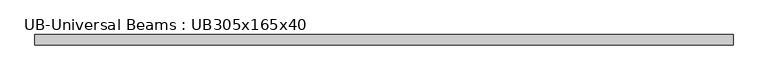
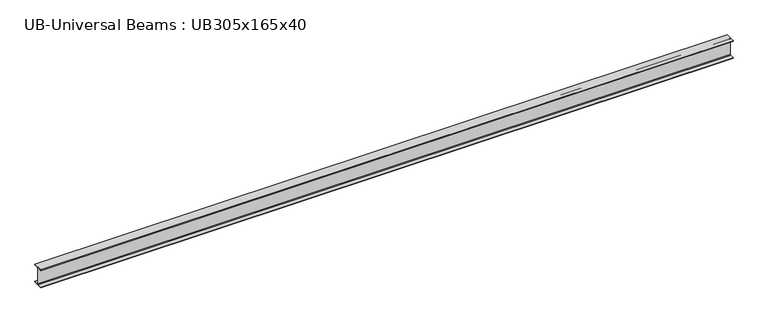
"""IFC4 building model written with IfcOpenShell, lengths in millimetres: member geometry, UB-Universal Beams : UB305x165x40."""

from ifc_helpers import new_model, si_unit, point, frame, frame_2d, origin, place, context, project, spatial, polyline, circle_curve, trimmed, segment, composite_curve, outline, extrude, source, transform, mapped, element, save


def ub_universal_beams_ub305x165x40_49d98a2e(model_context):
    return source(origin(), model_context, "Body", "SweptSolid", [
        extrude(outline(composite_curve([segment(polyline([(82.5, -141.5), (82.5, -151.7), (-82.5, -151.7), (-82.5, -141.5), (-11.9, -141.5)]), True, "CONTINUOUS"), segment(trimmed(circle_curve(frame_2d((-11.9, -132.6)), 8.9), [point((-11.9, -141.5))], [point((-3.0, -132.6))], True, "CARTESIAN"), True, "CONTINUOUS"), segment(polyline([(-3.0, -132.6), (-3.0, 132.6)]), True, "CONTINUOUS"), segment(trimmed(circle_curve(frame_2d((-11.9, 132.6)), 8.9), [point((-3.0, 132.6))], [point((-11.9, 141.5))], True, "CARTESIAN"), True, "CONTINUOUS"), segment(polyline([(-11.9, 141.5), (-82.5, 141.5), (-82.5, 151.7), (82.5, 151.7), (82.5, 141.5), (11.9, 141.5)]), True, "CONTINUOUS"), segment(trimmed(circle_curve(frame_2d((11.9, 132.6)), 8.9), [point((11.9, 141.5))], [point((3.0, 132.6))], True, "CARTESIAN"), True, "CONTINUOUS"), segment(polyline([(3.0, 132.6), (3.0, -132.6)]), True, "CONTINUOUS"), segment(trimmed(circle_curve(frame_2d((11.9, -132.6)), 8.9), [point((3.0, -132.6))], [point((11.9, -141.5))], True, "CARTESIAN"), True, "CONTINUOUS"), segment(polyline([(11.9, -141.5), (82.5, -141.5)]), True, "CONTINUOUS")], self_intersect=False)), frame((-5634.8, 0.0, 0.0), z_axis=(1.0, 0.0, 0.0), x_axis=(0.0, 1.0, 0.0)), (0.0, 0.0, 1.0), 11256.5),
    ])


if __name__ == "__main__":
    model = new_model("IFC4")
    model_context = context("Model", 3, world=origin())
    ifc_project = project(units=[si_unit("LENGTHUNIT", "METRE", prefix="MILLI")], contexts=[model_context])
    site = spatial("IfcSite", under=ifc_project)
    building = spatial("IfcBuilding", under=site)
    placement = place(None, origin())
    ub_universal_beams_ub305x165x40_shape = ub_universal_beams_ub305x165x40_49d98a2e(model_context)
    element("IfcMember", 1, ObjectType="UB-Universal Beams : UB305x165x40", at=placement, inside=building, context=model_context, shape_type="MappedRepresentation", body=[
        mapped(ub_universal_beams_ub305x165x40_shape, transform((0.0, 0.0, 0.0), x_axis=(1.0, 0.0, 0.0), y_axis=(0.0, 1.0, 0.0), z_axis=(0.0, 0.0, 1.0))),
    ])
    save(model, "model.ifc")

# Revit data of these elements
# Type "UB-Universal Beams : UB305x165x40"
#   Section Name Key = "UB305X165X40"
#   Width = 16.5 cm
#   Web Thickness = 0.6 cm
#   Web Fillet = 0.89 cm
#   Warping Constant = 164000.0 cm⁶
#   Torsional Moment of Inertia = 14.70 cm⁴
#   Section Area = 51.3 cm²
#   Plastic Modulus weak axis = 142.0 cm³
#   Plastic Modulus strong axis = 623.0 cm³
#   Nominal Weight = 40.2999 kgf/m
#   Moment of Inertia weak axis = 764.00 cm⁴
#   Moment of Inertia strong axis = 8503.00 cm⁴
#   Height = 30.34 cm
#   Flange Thickness = 1.02 cm
#   Elastic Modulus weak axis = 92.6 cm³
#   Elastic Modulus strong axis = 560.0 cm³
#   Centroid Vertical = 15.17 cm
#   Centroid Horizontal = 8.25 cm
#   Bolt Spacing = 9.0 cm
#   Length [instance default] = 1500 mm
#   Structural Material [instance default] = Metal - Steel 43-275
#   Type Comments = ""
#   Assembly Code = ""
# Element 1 (IfcMember, "UB-Universal Beams : UB305x165x40")
#   Materials on its faces: "Metal - Steel 43-275"
# Materials
#   "Metal - Steel 43-275": class "Metal", colour RGB 247 247 247, transparency 0, Cost = 0
